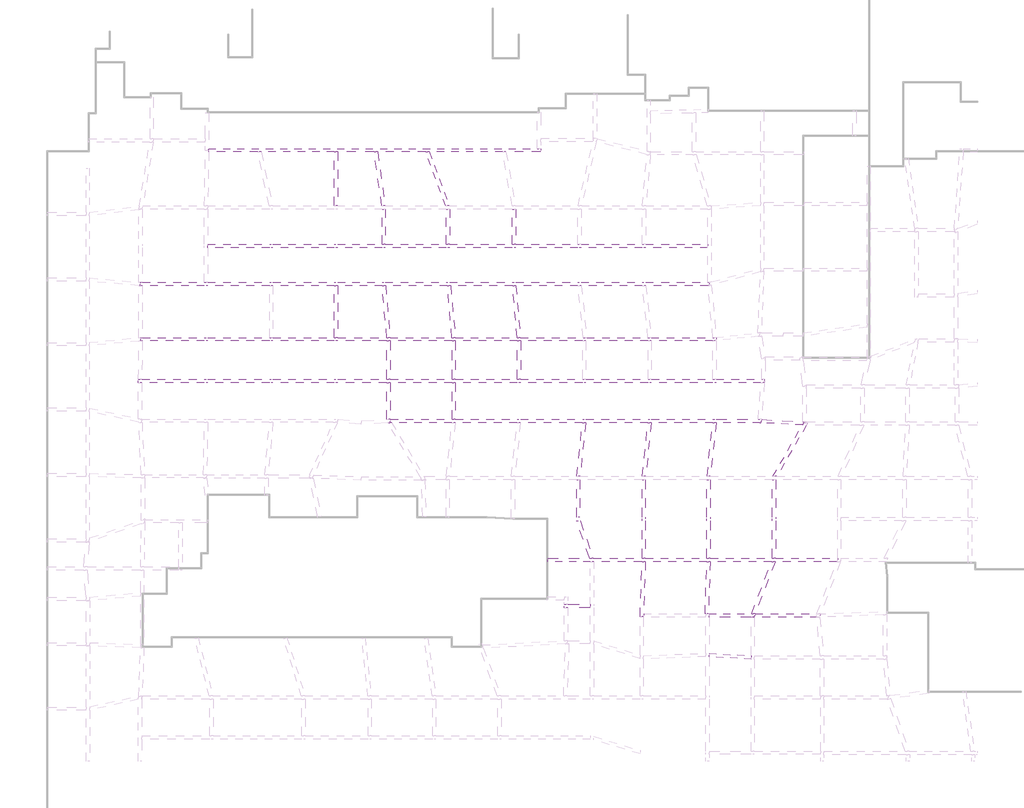
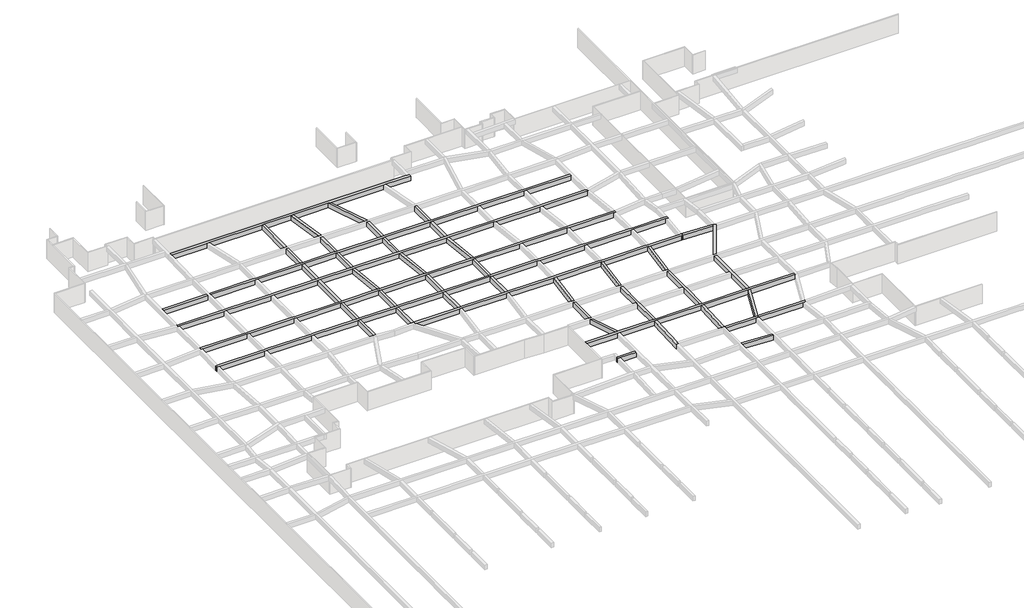
# One storey, part 36 of 45: 39 beams.
"""IFC4 building model written with IfcOpenShell, lengths in millimetres."""

from ifc_helpers import new_model, si_unit, frame, origin, place, context, project, spatial, polyline, outline, extrude, faceted_brep, element, save

model = new_model("IFC4")

# Units and contexts
model_context = context("Model", 3, world=origin())
ifc_project = project(units=[si_unit("LENGTHUNIT", "METRE", prefix="MILLI")], contexts=[model_context])

# Site, building, storey
site = spatial("IfcSite", under=ifc_project)
building = spatial("IfcBuilding", under=site)
storey = spatial("IfcBuildingStorey", under=building, Name="户型图", Elevation=0.0)

# Beams
placement = place(None, origin())
element("IfcBeam", 1, ObjectType="混凝土 - 矩形梁 : KL_beam", at=placement, inside=storey, context=model_context, shape_type="SweptSolid", body=[
    extrude(outline(polyline([(-120360.6744654, 184740.2921988), (-120760.6744654, 184740.2921988), (-120760.6744654, 191179.2504337), (-120360.6744654, 191179.2504337), (-120360.6744654, 184740.2921988)])), frame((0.0, 0.0, 2500.0), z_axis=(0.0, 0.0, 1.0), x_axis=(1.0, 0.0, 0.0)), (0.0, 0.0, 1.0), 800.0),
])
element("IfcBeam", 2, ObjectType="混凝土 - 矩形梁 : KL_beam", at=placement, inside=storey, context=model_context, shape_type="SweptSolid", body=[
    extrude(outline(polyline([(-114686.8171178, 184740.2921988), (-115090.7481468, 184740.2921988), (-115995.6847118, 191179.2504337), (-115591.7536828, 191179.2504337), (-114686.8171178, 184740.2921988)])), frame((0.0, 0.0, 2500.0), z_axis=(0.0, 0.0, 1.0), x_axis=(1.0, 0.0, 0.0)), (0.0, 0.0, 1.0), 800.0),
])
element("IfcBeam", 3, ObjectType="混凝土 - 矩形梁 : KL_beam", at=placement, inside=storey, context=model_context, shape_type="SweptSolid", body=[
    extrude(outline(polyline([(-107060.4801488, 184740.2921988), (-107486.1512578, 184740.2921988), (-109829.740395, 191179.2504337), (-109404.069286, 191179.2504337), (-107060.4801488, 184740.2921988)])), frame((0.0, 0.0, 2500.0), z_axis=(0.0, 0.0, 1.0), x_axis=(1.0, 0.0, 0.0)), (0.0, 0.0, 1.0), 800.0),
])
element("IfcBeam", 4, ObjectType="混凝土 - 矩形梁 : KL_beam", at=placement, inside=storey, context=model_context, shape_type="Brep", body=[
    faceted_brep([(-76031.325523, 175615.3210168, 3300.0), (-76160.6744654, 175615.3210168, 3300.0), (-83597.2475165, 175615.3210168, 3300.0), (-83997.2475165, 175615.3210168, 3300.0), (-91300.5216564, 175615.3210168, 3300.0), (-91700.5216564, 175615.3210168, 3300.0), (-99100.5216564, 175615.3210168, 3300.0), (-99500.5216564, 175615.3210168, 3300.0), (-107000.5216564, 175615.3210168, 3300.0), (-107400.5216564, 175615.3210168, 3300.0), (-114660.6744654, 175615.3210168, 3300.0), (-115060.6744654, 175615.3210168, 3300.0), (-120360.6744654, 175615.3210168, 3300.0), (-120760.6744654, 175615.3210168, 3300.0), (-128080.5216564, 175615.3210168, 3300.0), (-128480.5216564, 175615.3210168, 3300.0), (-135860.6744654, 175615.3210168, 3300.0), (-136260.6744654, 175615.3210168, 3300.0), (-143669.0135418, 175615.3210168, 3300.0), (-143895.9184786, 175615.3210168, 3300.0), (-143913.3828558, 175215.3210168, 3300.0), (-143669.0135418, 175215.3210168, 3300.0), (-136260.6744654, 175215.3210168, 3300.0), (-135860.6744654, 175215.3210168, 3300.0), (-128480.5216564, 175215.3210168, 3300.0), (-128080.5216564, 175215.3210168, 3300.0), (-120760.6744654, 175215.3210168, 3300.0), (-120360.6744654, 175215.3210168, 3300.0), (-115043.6071944, 175215.3210168, 3300.0), (-114642.0148509, 175215.3210168, 3300.0), (-107271.1801788, 175215.3210168, 3300.0), (-106869.5878353, 175215.3210168, 3300.0), (-99483.7878912, 175215.3210168, 3300.0), (-99082.2599562, 175215.3210168, 3300.0), (-91680.6024653, 175215.3210168, 3300.0), (-91278.3991535, 175215.3210168, 3300.0), (-83977.3283253, 175215.3210168, 3300.0), (-83575.1250135, 175215.3210168, 3300.0), (-76142.4560482, 175215.3210168, 3300.0), (-75977.9758113, 175215.3210168, 3300.0), (-143913.3828558, 175215.3210168, 2500.0), (-143669.0135418, 175215.3210168, 2500.0), (-136260.6744654, 175215.3210168, 2500.0), (-135860.6744654, 175215.3210168, 2500.0), (-128480.5216564, 175215.3210168, 2500.0), (-128080.5216564, 175215.3210168, 2500.0), (-120760.6744654, 175215.3210168, 2500.0), (-120360.6744654, 175215.3210168, 2500.0), (-115043.6071944, 175215.3210168, 2500.0), (-114642.0148509, 175215.3210168, 2500.0), (-107271.1801788, 175215.3210168, 2500.0), (-106869.5878353, 175215.3210168, 2500.0), (-99483.7878912, 175215.3210168, 2500.0), (-99082.2599562, 175215.3210168, 2500.0), (-91680.6024653, 175215.3210168, 2500.0), (-91278.3991535, 175215.3210168, 2500.0), (-83977.3283253, 175215.3210168, 2500.0), (-83575.1250135, 175215.3210168, 2500.0), (-76142.4560482, 175215.3210168, 2500.0), (-75977.9758113, 175215.3210168, 2500.0), (-143895.9184786, 175615.3210168, 2500.0), (-143669.0135418, 175615.3210168, 2500.0), (-136260.6744654, 175615.3210168, 2500.0), (-135860.6744654, 175615.3210168, 2500.0), (-128480.5216564, 175615.3210168, 2500.0), (-128080.5216564, 175615.3210168, 2500.0), (-120760.6744654, 175615.3210168, 2500.0), (-120360.6744654, 175615.3210168, 2500.0), (-115060.6744654, 175615.3210168, 2500.0), (-114660.6744654, 175615.3210168, 2500.0), (-107400.5216564, 175615.3210168, 2500.0), (-107000.5216564, 175615.3210168, 2500.0), (-99500.5216564, 175615.3210168, 2500.0), (-99100.5216564, 175615.3210168, 2500.0), (-91700.5216564, 175615.3210168, 2500.0), (-91300.5216564, 175615.3210168, 2500.0), (-83997.2475165, 175615.3210168, 2500.0), (-83597.2475165, 175615.3210168, 2500.0), (-76160.6744654, 175615.3210168, 2500.0), (-76031.325523, 175615.3210168, 2500.0)], [[[0, 1, 2, 3, 4, 5, 6, 7, 8, 9, 10, 11, 12, 13, 14, 15, 16, 17, 18, 19, 20, 21, 22, 23, 24, 25, 26, 27, 28, 29, 30, 31, 32, 33, 34, 35, 36, 37, 38, 39]], [[39, 38, 37, 36, 35, 34, 33, 32, 31, 30, 29, 28, 27, 26, 25, 24, 23, 22, 21, 20, 40, 41, 42, 43, 44, 45, 46, 47, 48, 49, 50, 51, 52, 53, 54, 55, 56, 57, 58, 59]], [[59, 58, 57, 56, 55, 54, 53, 52, 51, 50, 49, 48, 47, 46, 45, 44, 43, 42, 41, 40, 60, 61, 62, 63, 64, 65, 66, 67, 68, 69, 70, 71, 72, 73, 74, 75, 76, 77, 78, 79]], [[19, 18, 17, 16, 15, 14, 13, 12, 11, 10, 9, 8, 7, 6, 5, 4, 3, 2, 1, 0, 79, 78, 77, 76, 75, 74, 73, 72, 71, 70, 69, 68, 67, 66, 65, 64, 63, 62, 61, 60]], [[19, 60, 40, 20]], [[0, 39, 59, 79]]]),
])
element("IfcBeam", 5, ObjectType="混凝土 - 矩形梁 : KL_beam", at=placement, inside=storey, context=model_context, shape_type="Brep", body=[
    faceted_brep([(-75186.161196, 169035.1135794, 3300.0), (-75587.7690547, 169035.1135794, 3300.0), (-82925.559037, 169035.1135794, 3300.0), (-83327.7623488, 169035.1135794, 3300.0), (-90628.833177, 169035.1135794, 3300.0), (-91031.0364888, 169035.1135794, 3300.0), (-98541.5618672, 169035.1135794, 3300.0), (-98943.0898022, 169035.1135794, 3300.0), (-106317.5889274, 169035.1135794, 3300.0), (-106719.1812709, 169035.1135794, 3300.0), (-114090.0159431, 169035.1135794, 3300.0), (-114491.6082865, 169035.1135794, 3300.0), (-120360.6744654, 169035.1135794, 3300.0), (-120760.6744654, 169035.1135794, 3300.0), (-128080.5216564, 169035.1135794, 3300.0), (-128480.5216564, 169035.1135794, 3300.0), (-135860.6744654, 169035.1135794, 3300.0), (-136260.6744654, 169035.1135794, 3300.0), (-143669.0135418, 169035.1135794, 3300.0), (-143878.581976, 169035.1135794, 3300.0), (-143859.4474089, 168635.1135794, 3300.0), (-143671.4793509, 168635.1135794, 3300.0), (-136260.6744654, 168635.1135794, 3300.0), (-135860.6744654, 168635.1135794, 3300.0), (-128480.5216564, 168635.1135794, 3300.0), (-128080.5216564, 168635.1135794, 3300.0), (-120760.6744654, 168635.1135794, 3300.0), (-120360.6744654, 168635.1135794, 3300.0), (-114472.9294157, 168635.1135794, 3300.0), (-114072.9294157, 168635.1135794, 3300.0), (-106700.5216564, 168635.1135794, 3300.0), (-106300.5216564, 168635.1135794, 3300.0), (-98924.7994609, 168635.1135794, 3300.0), (-98524.7994609, 168635.1135794, 3300.0), (-91124.7994609, 168635.1135794, 3300.0), (-90724.7994609, 168635.1135794, 3300.0), (-83305.6398459, 168635.1135794, 3300.0), (-82905.6398459, 168635.1135794, 3300.0), (-75569.0146925, 168635.1135794, 3300.0), (-75358.5331366, 168635.1135794, 3300.0), (-75186.161196, 168635.1135794, 3300.0), (-75186.161196, 168653.2306004, 3300.0), (-143859.4474089, 168635.1135794, 2500.0), (-143671.4793509, 168635.1135794, 2500.0), (-136260.6744654, 168635.1135794, 2500.0), (-135860.6744654, 168635.1135794, 2500.0), (-128480.5216564, 168635.1135794, 2500.0), (-128080.5216564, 168635.1135794, 2500.0), (-120760.6744654, 168635.1135794, 2500.0), (-120360.6744654, 168635.1135794, 2500.0), (-114472.9294157, 168635.1135794, 2500.0), (-114072.9294157, 168635.1135794, 2500.0), (-106700.5216564, 168635.1135794, 2500.0), (-106300.5216564, 168635.1135794, 2500.0), (-98924.7994609, 168635.1135794, 2500.0), (-98524.7994609, 168635.1135794, 2500.0), (-91124.7994609, 168635.1135794, 2500.0), (-90724.7994609, 168635.1135794, 2500.0), (-83305.6398459, 168635.1135794, 2500.0), (-82905.6398459, 168635.1135794, 2500.0), (-75569.0146925, 168635.1135794, 2500.0), (-75358.5331366, 168635.1135794, 2500.0), (-75186.161196, 168635.1135794, 2500.0), (-143878.581976, 169035.1135794, 2500.0), (-143669.0135418, 169035.1135794, 2500.0), (-136260.6744654, 169035.1135794, 2500.0), (-135860.6744654, 169035.1135794, 2500.0), (-128480.5216564, 169035.1135794, 2500.0), (-128080.5216564, 169035.1135794, 2500.0), (-120760.6744654, 169035.1135794, 2500.0), (-120360.6744654, 169035.1135794, 2500.0), (-114491.6082865, 169035.1135794, 2500.0), (-114090.0159431, 169035.1135794, 2500.0), (-106719.1812709, 169035.1135794, 2500.0), (-106317.5889274, 169035.1135794, 2500.0), (-98943.0898022, 169035.1135794, 2500.0), (-98541.5618672, 169035.1135794, 2500.0), (-91031.0364888, 169035.1135794, 2500.0), (-90628.833177, 169035.1135794, 2500.0), (-83327.7623488, 169035.1135794, 2500.0), (-82925.559037, 169035.1135794, 2500.0), (-75587.7690547, 169035.1135794, 2500.0), (-75186.161196, 169035.1135794, 2500.0), (-75186.161196, 168653.2306004, 2500.0)], [[[0, 1, 2, 3, 4, 5, 6, 7, 8, 9, 10, 11, 12, 13, 14, 15, 16, 17, 18, 19, 20, 21, 22, 23, 24, 25, 26, 27, 28, 29, 30, 31, 32, 33, 34, 35, 36, 37, 38, 39, 40, 41]], [[40, 39, 38, 37, 36, 35, 34, 33, 32, 31, 30, 29, 28, 27, 26, 25, 24, 23, 22, 21, 20, 42, 43, 44, 45, 46, 47, 48, 49, 50, 51, 52, 53, 54, 55, 56, 57, 58, 59, 60, 61, 62]], [[62, 61, 60, 59, 58, 57, 56, 55, 54, 53, 52, 51, 50, 49, 48, 47, 46, 45, 44, 43, 42, 63, 64, 65, 66, 67, 68, 69, 70, 71, 72, 73, 74, 75, 76, 77, 78, 79, 80, 81, 82, 83]], [[19, 18, 17, 16, 15, 14, 13, 12, 11, 10, 9, 8, 7, 6, 5, 4, 3, 2, 1, 0, 82, 81, 80, 79, 78, 77, 76, 75, 74, 73, 72, 71, 70, 69, 68, 67, 66, 65, 64, 63]], [[19, 63, 42, 20]], [[0, 41, 40, 62, 83, 82]]]),
])
element("IfcBeam", 6, ObjectType="混凝土 - 矩形梁 : KL_beam", at=placement, inside=storey, context=model_context, shape_type="Brep", body=[
    faceted_brep([(-69444.6043733, 163650.6823883, 3300.0), (-69444.6043733, 163735.2368527, 3300.0), (-69444.6043733, 164050.6823883, 3300.0), (-69744.9443936, 164050.6823883, 3300.0), (-75169.0146925, 164050.6823883, 3300.0), (-75569.0146925, 164050.6823883, 3300.0), (-82905.6398459, 164050.6823883, 3300.0), (-83305.6398459, 164050.6823883, 3300.0), (-90724.7994609, 164050.6823883, 3300.0), (-91124.7994609, 164050.6823883, 3300.0), (-98524.7994609, 164050.6823883, 3300.0), (-98924.7994609, 164050.6823883, 3300.0), (-106300.5216564, 164050.6823883, 3300.0), (-106700.5216564, 164050.6823883, 3300.0), (-114072.9294157, 164050.6823883, 3300.0), (-114472.9294157, 164050.6823883, 3300.0), (-120360.6744654, 164050.6823883, 3300.0), (-120760.6744654, 164050.6823883, 3300.0), (-128080.5216564, 164050.6823883, 3300.0), (-128480.5216564, 164050.6823883, 3300.0), (-135860.6744654, 164050.6823883, 3300.0), (-136260.6744654, 164050.6823883, 3300.0), (-143728.3270835, 164050.6823883, 3300.0), (-144128.3578352, 164050.6823883, 3300.0), (-144130.8224936, 164050.6823883, 3300.0), (-144130.8224936, 163650.6823883, 3300.0), (-143730.8224936, 163650.6823883, 3300.0), (-136260.6744654, 163650.6823883, 3300.0), (-135860.6744654, 163650.6823883, 3300.0), (-128480.5216564, 163650.6823883, 3300.0), (-128080.5216564, 163650.6823883, 3300.0), (-120760.6744654, 163650.6823883, 3300.0), (-120360.6744654, 163650.6823883, 3300.0), (-114472.9294157, 163650.6823883, 3300.0), (-114072.9294157, 163650.6823883, 3300.0), (-106700.5216564, 163650.6823883, 3300.0), (-106300.5216564, 163650.6823883, 3300.0), (-98924.7994609, 163650.6823883, 3300.0), (-98524.7994609, 163650.6823883, 3300.0), (-91124.7994609, 163650.6823883, 3300.0), (-90724.7994609, 163650.6823883, 3300.0), (-83305.6398459, 163650.6823883, 3300.0), (-82905.6398459, 163650.6823883, 3300.0), (-75569.0146925, 163650.6823883, 3300.0), (-75169.0146925, 163650.6823883, 3300.0), (-69845.6243611, 163650.6823883, 3300.0), (-69444.6043733, 163650.6823883, 2500.0), (-144130.8224936, 163650.6823883, 2500.0), (-143730.8224936, 163650.6823883, 2500.0), (-136260.6744654, 163650.6823883, 2500.0), (-135860.6744654, 163650.6823883, 2500.0), (-128480.5216564, 163650.6823883, 2500.0), (-128080.5216564, 163650.6823883, 2500.0), (-120760.6744654, 163650.6823883, 2500.0), (-120360.6744654, 163650.6823883, 2500.0), (-114472.9294157, 163650.6823883, 2500.0), (-114072.9294157, 163650.6823883, 2500.0), (-106700.5216564, 163650.6823883, 2500.0), (-106300.5216564, 163650.6823883, 2500.0), (-98924.7994609, 163650.6823883, 2500.0), (-98524.7994609, 163650.6823883, 2500.0), (-91124.7994609, 163650.6823883, 2500.0), (-90724.7994609, 163650.6823883, 2500.0), (-83305.6398459, 163650.6823883, 2500.0), (-82905.6398459, 163650.6823883, 2500.0), (-75569.0146925, 163650.6823883, 2500.0), (-75169.0146925, 163650.6823883, 2500.0), (-69845.6243611, 163650.6823883, 2500.0), (-69444.6043733, 164050.6823883, 2500.0), (-69444.6043733, 163735.2368527, 2500.0), (-144130.8224936, 164050.6823883, 2500.0), (-144128.3578352, 164050.6823883, 2500.0), (-143728.3270835, 164050.6823883, 2500.0), (-136260.6744654, 164050.6823883, 2500.0), (-135860.6744654, 164050.6823883, 2500.0), (-128480.5216564, 164050.6823883, 2500.0), (-128080.5216564, 164050.6823883, 2500.0), (-120760.6744654, 164050.6823883, 2500.0), (-120360.6744654, 164050.6823883, 2500.0), (-114472.9294157, 164050.6823883, 2500.0), (-114072.9294157, 164050.6823883, 2500.0), (-106700.5216564, 164050.6823883, 2500.0), (-106300.5216564, 164050.6823883, 2500.0), (-98924.7994609, 164050.6823883, 2500.0), (-98524.7994609, 164050.6823883, 2500.0), (-91124.7994609, 164050.6823883, 2500.0), (-90724.7994609, 164050.6823883, 2500.0), (-83305.6398459, 164050.6823883, 2500.0), (-82905.6398459, 164050.6823883, 2500.0), (-75569.0146925, 164050.6823883, 2500.0), (-75169.0146925, 164050.6823883, 2500.0), (-69744.9443936, 164050.6823883, 2500.0)], [[[0, 1, 2, 3, 4, 5, 6, 7, 8, 9, 10, 11, 12, 13, 14, 15, 16, 17, 18, 19, 20, 21, 22, 23, 24, 25, 26, 27, 28, 29, 30, 31, 32, 33, 34, 35, 36, 37, 38, 39, 40, 41, 42, 43, 44, 45]], [[46, 0, 45, 44, 43, 42, 41, 40, 39, 38, 37, 36, 35, 34, 33, 32, 31, 30, 29, 28, 27, 26, 25, 47, 48, 49, 50, 51, 52, 53, 54, 55, 56, 57, 58, 59, 60, 61, 62, 63, 64, 65, 66, 67]], [[68, 69, 46, 67, 66, 65, 64, 63, 62, 61, 60, 59, 58, 57, 56, 55, 54, 53, 52, 51, 50, 49, 48, 47, 70, 71, 72, 73, 74, 75, 76, 77, 78, 79, 80, 81, 82, 83, 84, 85, 86, 87, 88, 89, 90, 91]], [[2, 68, 91, 90, 89, 88, 87, 86, 85, 84, 83, 82, 81, 80, 79, 78, 77, 76, 75, 74, 73, 72, 71, 70, 24, 23, 22, 21, 20, 19, 18, 17, 16, 15, 14, 13, 12, 11, 10, 9, 8, 7, 6, 5, 4, 3]], [[25, 24, 70, 47]], [[2, 1, 0, 46, 69, 68]]]),
])
element("IfcBeam", 7, ObjectType="混凝土 - 矩形梁 : KL_beam", at=placement, inside=storey, context=model_context, shape_type="Brep", body=[
    faceted_brep([(-143669.0135418, 180177.2946529, 3300.0), (-143669.0135418, 179777.2946529, 3300.0), (-136260.6744654, 179777.2946529, 3300.0), (-136260.6744654, 180177.2946529, 3300.0), (-143669.0135418, 179777.2946529, 2500.0), (-136260.6744654, 179777.2946529, 2500.0), (-143669.0135418, 180177.2946529, 2500.0), (-136260.6744654, 180177.2946529, 2500.0)], [[[0, 1, 2, 3]], [[1, 4, 5, 2]], [[4, 6, 7, 5]], [[6, 0, 3, 7]], [[1, 0, 6, 4]], [[3, 2, 5, 7]]]),
    faceted_brep([(-135860.6744654, 179777.2946529, 3300.0), (-135860.6744654, 180177.2946529, 3300.0), (-135860.6744654, 180177.2946529, 2500.0), (-135860.6744654, 179777.2946529, 2500.0), (-128480.5216564, 179777.2946529, 3300.0), (-128080.5216564, 179777.2946529, 3300.0), (-120760.6744654, 179777.2946529, 3300.0), (-120360.6744654, 179777.2946529, 3300.0), (-115060.6744654, 179777.2946529, 3300.0), (-114660.6744654, 179777.2946529, 3300.0), (-107400.5216564, 179777.2946529, 3300.0), (-107000.5216564, 179777.2946529, 3300.0), (-99500.5216564, 179777.2946529, 3300.0), (-99100.5216564, 179777.2946529, 3300.0), (-91700.5216564, 179777.2946529, 3300.0), (-91300.5216564, 179777.2946529, 3300.0), (-83997.2475165, 179777.2946529, 3300.0), (-83597.2475165, 179777.2946529, 3300.0), (-76160.6744654, 179777.2946529, 3300.0), (-76160.6744654, 180177.2946529, 3300.0), (-83597.2475165, 180177.2946529, 3300.0), (-83997.2475165, 180177.2946529, 3300.0), (-91300.5216564, 180177.2946529, 3300.0), (-91700.5216564, 180177.2946529, 3300.0), (-99100.5216564, 180177.2946529, 3300.0), (-99500.5216564, 180177.2946529, 3300.0), (-107000.5216564, 180177.2946529, 3300.0), (-107400.5216564, 180177.2946529, 3300.0), (-114660.6744654, 180177.2946529, 3300.0), (-115060.6744654, 180177.2946529, 3300.0), (-120360.6744654, 180177.2946529, 3300.0), (-120760.6744654, 180177.2946529, 3300.0), (-128080.5216564, 180177.2946529, 3300.0), (-128480.5216564, 180177.2946529, 3300.0), (-128480.5216564, 179777.2946529, 2500.0), (-128080.5216564, 179777.2946529, 2500.0), (-120760.6744654, 179777.2946529, 2500.0), (-120360.6744654, 179777.2946529, 2500.0), (-115060.6744654, 179777.2946529, 2500.0), (-114660.6744654, 179777.2946529, 2500.0), (-107400.5216564, 179777.2946529, 2500.0), (-107000.5216564, 179777.2946529, 2500.0), (-99500.5216564, 179777.2946529, 2500.0), (-99100.5216564, 179777.2946529, 2500.0), (-91700.5216564, 179777.2946529, 2500.0), (-91300.5216564, 179777.2946529, 2500.0), (-83997.2475165, 179777.2946529, 2500.0), (-83597.2475165, 179777.2946529, 2500.0), (-76160.6744654, 179777.2946529, 2500.0), (-128480.5216564, 180177.2946529, 2500.0), (-128080.5216564, 180177.2946529, 2500.0), (-120760.6744654, 180177.2946529, 2500.0), (-120360.6744654, 180177.2946529, 2500.0), (-115060.6744654, 180177.2946529, 2500.0), (-114660.6744654, 180177.2946529, 2500.0), (-107400.5216564, 180177.2946529, 2500.0), (-107000.5216564, 180177.2946529, 2500.0), (-99500.5216564, 180177.2946529, 2500.0), (-99100.5216564, 180177.2946529, 2500.0), (-91700.5216564, 180177.2946529, 2500.0), (-91300.5216564, 180177.2946529, 2500.0), (-83997.2475165, 180177.2946529, 2500.0), (-83597.2475165, 180177.2946529, 2500.0), (-76160.6744654, 180177.2946529, 2500.0)], [[[0, 1, 2, 3]], [[1, 0, 4, 5, 6, 7, 8, 9, 10, 11, 12, 13, 14, 15, 16, 17, 18, 19, 20, 21, 22, 23, 24, 25, 26, 27, 28, 29, 30, 31, 32, 33]], [[0, 3, 34, 35, 36, 37, 38, 39, 40, 41, 42, 43, 44, 45, 46, 47, 48, 18, 17, 16, 15, 14, 13, 12, 11, 10, 9, 8, 7, 6, 5, 4]], [[3, 2, 49, 50, 51, 52, 53, 54, 55, 56, 57, 58, 59, 60, 61, 62, 63, 48, 47, 46, 45, 44, 43, 42, 41, 40, 39, 38, 37, 36, 35, 34]], [[2, 1, 33, 32, 31, 30, 29, 28, 27, 26, 25, 24, 23, 22, 21, 20, 19, 63, 62, 61, 60, 59, 58, 57, 56, 55, 54, 53, 52, 51, 50, 49]], [[19, 18, 48, 63]]]),
])
element("IfcBeam", 8, ObjectType="混凝土 - 矩形梁 : KL_beam", at=placement, inside=storey, context=model_context, shape_type="SweptSolid", body=[
    extrude(outline(polyline([(-120760.6744654, 184340.2921988), (-120360.6744654, 184340.2921988), (-120360.6744654, 180177.2946529), (-120760.6744654, 180177.2946529), (-120760.6744654, 184340.2921988)])), frame((0.0, 0.0, 2500.0), z_axis=(0.0, 0.0, 1.0), x_axis=(1.0, 0.0, 0.0)), (0.0, 0.0, 1.0), 800.0),
    extrude(outline(polyline([(-120360.6744654, 159299.3775215), (-120760.6744654, 159299.3775215), (-120760.6744654, 163650.6823883), (-120360.6744654, 163650.6823883), (-120360.6744654, 159299.3775215)])), frame((0.0, 0.0, 2500.0), z_axis=(0.0, 0.0, 1.0), x_axis=(1.0, 0.0, 0.0)), (0.0, 0.0, 1.0), 800.0),
    extrude(outline(polyline([(-120760.6744654, 175215.3210168), (-120360.6744654, 175215.3210168), (-120360.6744654, 169035.1135794), (-120760.6744654, 169035.1135794), (-120760.6744654, 175215.3210168)])), frame((0.0, 0.0, 2500.0), z_axis=(0.0, 0.0, 1.0), x_axis=(1.0, 0.0, 0.0)), (0.0, 0.0, 1.0), 800.0),
    extrude(outline(polyline([(-120360.6744654, 175615.3210168), (-120760.6744654, 175615.3210168), (-120760.6744654, 179777.2946529), (-120360.6744654, 179777.2946529), (-120360.6744654, 175615.3210168)])), frame((0.0, 0.0, 2500.0), z_axis=(0.0, 0.0, 1.0), x_axis=(1.0, 0.0, 0.0)), (0.0, 0.0, 1.0), 800.0),
    extrude(outline(polyline([(-120760.6744654, 168635.1135794), (-120360.6744654, 168635.1135794), (-120360.6744654, 164050.6823883), (-120760.6744654, 164050.6823883), (-120760.6744654, 168635.1135794)])), frame((0.0, 0.0, 2500.0), z_axis=(0.0, 0.0, 1.0), x_axis=(1.0, 0.0, 0.0)), (0.0, 0.0, 1.0), 800.0),
])
element("IfcBeam", 9, ObjectType="混凝土 - 矩形梁 : KL_beam", at=placement, inside=storey, context=model_context, shape_type="SweptSolid", body=[
    extrude(outline(polyline([(-114072.9294157, 159273.5727809), (-114472.9294157, 159252.6096692), (-114472.9294157, 163650.6823883), (-114072.9294157, 163650.6823883), (-114072.9294157, 159273.5727809)])), frame((0.0, 0.0, 2500.0), z_axis=(0.0, 0.0, 1.0), x_axis=(1.0, 0.0, 0.0)), (0.0, 0.0, 1.0), 800.0),
])
element("IfcBeam", 10, ObjectType="混凝土 - 矩形梁 : KL_beam", at=placement, inside=storey, context=model_context, shape_type="SweptSolid", body=[
    extrude(outline(polyline([(-114472.9294157, 168635.1135794), (-114072.9294157, 168635.1135794), (-114072.9294157, 164050.6823883), (-114472.9294157, 164050.6823883), (-114472.9294157, 168635.1135794)])), frame((0.0, 0.0, 2500.0), z_axis=(0.0, 0.0, 1.0), x_axis=(1.0, 0.0, 0.0)), (0.0, 0.0, 1.0), 800.0),
])
element("IfcBeam", 11, ObjectType="混凝土 - 矩形梁 : KL_beam", at=placement, inside=storey, context=model_context, shape_type="SweptSolid", body=[
    extrude(outline(polyline([(-115060.6744654, 184340.2921988), (-114660.6744654, 184340.2921988), (-114660.6744654, 180177.2946529), (-115060.6744654, 180177.2946529), (-115060.6744654, 184340.2921988)])), frame((0.0, 0.0, 2500.0), z_axis=(0.0, 0.0, 1.0), x_axis=(1.0, 0.0, 0.0)), (0.0, 0.0, 1.0), 800.0),
    extrude(outline(polyline([(-114660.6744654, 175615.3210168), (-115060.6744654, 175615.3210168), (-115060.6744654, 179777.2946529), (-114660.6744654, 179777.2946529), (-114660.6744654, 175615.3210168)])), frame((0.0, 0.0, 2500.0), z_axis=(0.0, 0.0, 1.0), x_axis=(1.0, 0.0, 0.0)), (0.0, 0.0, 1.0), 800.0),
])
element("IfcBeam", 12, ObjectType="混凝土 - 矩形梁 : KL_beam", at=placement, inside=storey, context=model_context, shape_type="SweptSolid", body=[
    extrude(outline(polyline([(-115043.6071944, 175215.3210168), (-114642.0148509, 175215.3210168), (-114090.0159431, 169035.1135794), (-114491.6082865, 169035.1135794), (-115043.6071944, 175215.3210168)])), frame((0.0, 0.0, 2500.0), z_axis=(0.0, 0.0, 1.0), x_axis=(1.0, 0.0, 0.0)), (0.0, 0.0, 1.0), 800.0),
])
element("IfcBeam", 13, ObjectType="混凝土 - 矩形梁 : KL_beam", at=placement, inside=storey, context=model_context, shape_type="SweptSolid", body=[
    extrude(outline(polyline([(-107400.5216564, 184340.2921988), (-107000.5216564, 184340.2921988), (-107000.5216564, 180177.2946529), (-107400.5216564, 180177.2946529), (-107400.5216564, 184340.2921988)])), frame((0.0, 0.0, 2500.0), z_axis=(0.0, 0.0, 1.0), x_axis=(1.0, 0.0, 0.0)), (0.0, 0.0, 1.0), 800.0),
    extrude(outline(polyline([(-107000.5216564, 175615.3210168), (-107400.5216564, 175615.3210168), (-107400.5216564, 179777.2946529), (-107000.5216564, 179777.2946529), (-107000.5216564, 175615.3210168)])), frame((0.0, 0.0, 2500.0), z_axis=(0.0, 0.0, 1.0), x_axis=(1.0, 0.0, 0.0)), (0.0, 0.0, 1.0), 800.0),
])
element("IfcBeam", 14, ObjectType="混凝土 - 矩形梁 : KL_beam", at=placement, inside=storey, context=model_context, shape_type="SweptSolid", body=[
    extrude(outline(polyline([(-107271.1801788, 175215.3210168), (-106869.5878353, 175215.3210168), (-106317.5889274, 169035.1135794), (-106719.1812709, 169035.1135794), (-107271.1801788, 175215.3210168)])), frame((0.0, 0.0, 2500.0), z_axis=(0.0, 0.0, 1.0), x_axis=(1.0, 0.0, 0.0)), (0.0, 0.0, 1.0), 800.0),
])
element("IfcBeam", 15, ObjectType="混凝土 - 矩形梁 : KL_beam", at=placement, inside=storey, context=model_context, shape_type="SweptSolid", body=[
    extrude(outline(polyline([(-106700.5216564, 168635.1135794), (-106300.5216564, 168635.1135794), (-106300.5216564, 164050.6823883), (-106700.5216564, 164050.6823883), (-106700.5216564, 168635.1135794)])), frame((0.0, 0.0, 2500.0), z_axis=(0.0, 0.0, 1.0), x_axis=(1.0, 0.0, 0.0)), (0.0, 0.0, 1.0), 800.0),
])
element("IfcBeam", 16, ObjectType="混凝土 - 矩形梁 : KL_beam", at=placement, inside=storey, context=model_context, shape_type="SweptSolid", body=[
    extrude(outline(polyline([(-106700.5216564, 163650.6823883), (-106300.5216564, 163650.6823883), (-106300.5216564, 159263.2495721), (-106700.5216564, 159263.2495721), (-106700.5216564, 163650.6823883)])), frame((0.0, 0.0, 2500.0), z_axis=(0.0, 0.0, 1.0), x_axis=(1.0, 0.0, 0.0)), (0.0, 0.0, 1.0), 800.0),
])
element("IfcBeam", 17, ObjectType="混凝土 - 矩形梁 : KL_beam", at=placement, inside=storey, context=model_context, shape_type="Brep", body=[
    faceted_brep([(-114072.9294157, 159263.2495721, 3300.0), (-114072.9294157, 158873.0238425, 3300.0), (-114259.4336062, 158863.2495721, 3300.0), (-113919.6906746, 158863.2495721, 3300.0), (-106722.8306205, 158863.2495721, 3300.0), (-106320.5918899, 158863.2495721, 3300.0), (-98947.1541949, 158863.2495721, 3300.0), (-98544.9154643, 158863.2495721, 3300.0), (-91147.1541949, 158863.2495721, 3300.0), (-90744.9154643, 158863.2495721, 3300.0), (-83327.9488099, 158863.2495721, 3300.0), (-82925.7100793, 158863.2495721, 3300.0), (-75591.3694264, 158863.2495721, 3300.0), (-75189.1306958, 158863.2495721, 3300.0), (-69978.1666, 158863.2495721, 3300.0), (-69786.7112953, 158863.2495721, 3300.0), (-69758.9094454, 159252.3077299, 3300.0), (-69758.1275482, 159263.2495721, 3300.0), (-70159.147536, 159263.2495721, 3300.0), (-75169.0146925, 159263.2495721, 3300.0), (-75569.0146925, 159263.2495721, 3300.0), (-82905.6398459, 159263.2495721, 3300.0), (-83305.6398459, 159263.2495721, 3300.0), (-90724.7994609, 159263.2495721, 3300.0), (-91124.7994609, 159263.2495721, 3300.0), (-98524.7994609, 159263.2495721, 3300.0), (-98924.7994609, 159263.2495721, 3300.0), (-106300.5216564, 159263.2495721, 3300.0), (-106700.5216564, 159263.2495721, 3300.0), (-114259.4336062, 158863.2495721, 2500.0), (-113919.6906746, 158863.2495721, 2500.0), (-106722.8306205, 158863.2495721, 2500.0), (-106320.5918899, 158863.2495721, 2500.0), (-98947.1541949, 158863.2495721, 2500.0), (-98544.9154643, 158863.2495721, 2500.0), (-91147.1541949, 158863.2495721, 2500.0), (-90744.9154643, 158863.2495721, 2500.0), (-83327.9488099, 158863.2495721, 2500.0), (-82925.7100793, 158863.2495721, 2500.0), (-75591.3694264, 158863.2495721, 2500.0), (-75189.1306958, 158863.2495721, 2500.0), (-69978.1666, 158863.2495721, 2500.0), (-69786.7112953, 158863.2495721, 2500.0), (-114072.9294157, 158873.0238425, 2500.0), (-114072.9294157, 159263.2495721, 2500.0), (-106700.5216564, 159263.2495721, 2500.0), (-106300.5216564, 159263.2495721, 2500.0), (-98924.7994609, 159263.2495721, 2500.0), (-98524.7994609, 159263.2495721, 2500.0), (-91124.7994609, 159263.2495721, 2500.0), (-90724.7994609, 159263.2495721, 2500.0), (-83305.6398459, 159263.2495721, 2500.0), (-82905.6398459, 159263.2495721, 2500.0), (-75569.0146925, 159263.2495721, 2500.0), (-75169.0146925, 159263.2495721, 2500.0), (-70159.147536, 159263.2495721, 2500.0), (-69758.1275482, 159263.2495721, 2500.0), (-69758.9094454, 159252.3077299, 2500.0)], [[[0, 1, 2, 3, 4, 5, 6, 7, 8, 9, 10, 11, 12, 13, 14, 15, 16, 17, 18, 19, 20, 21, 22, 23, 24, 25, 26, 27, 28]], [[2, 29, 30, 31, 32, 33, 34, 35, 36, 37, 38, 39, 40, 41, 42, 15, 14, 13, 12, 11, 10, 9, 8, 7, 6, 5, 4, 3]], [[43, 44, 45, 46, 47, 48, 49, 50, 51, 52, 53, 54, 55, 56, 57, 42, 41, 40, 39, 38, 37, 36, 35, 34, 33, 32, 31, 30, 29]], [[44, 0, 28, 27, 26, 25, 24, 23, 22, 21, 20, 19, 18, 17, 56, 55, 54, 53, 52, 51, 50, 49, 48, 47, 46, 45]], [[43, 1, 0, 44]], [[1, 43, 29, 2]], [[17, 16, 15, 42, 57, 56]]]),
])
element("IfcBeam", 18, ObjectType="混凝土 - 矩形梁 : KL_beam", at=placement, inside=storey, context=model_context, shape_type="SweptSolid", body=[
    extrude(outline(polyline([(-99500.5216564, 184340.2921988), (-99100.5216564, 184340.2921988), (-99100.5216564, 180177.2946529), (-99500.5216564, 180177.2946529), (-99500.5216564, 184340.2921988)])), frame((0.0, 0.0, 2500.0), z_axis=(0.0, 0.0, 1.0), x_axis=(1.0, 0.0, 0.0)), (0.0, 0.0, 1.0), 800.0),
    extrude(outline(polyline([(-99100.5216564, 175615.3210168), (-99500.5216564, 175615.3210168), (-99500.5216564, 179777.2946529), (-99100.5216564, 179777.2946529), (-99100.5216564, 175615.3210168)])), frame((0.0, 0.0, 2500.0), z_axis=(0.0, 0.0, 1.0), x_axis=(1.0, 0.0, 0.0)), (0.0, 0.0, 1.0), 800.0),
])
element("IfcBeam", 19, ObjectType="混凝土 - 矩形梁 : KL_beam", at=placement, inside=storey, context=model_context, shape_type="SweptSolid", body=[
    extrude(outline(polyline([(-99483.7878912, 175215.3210168), (-99082.2599562, 175215.3210168), (-98541.5618672, 169035.1135794), (-98943.0898022, 169035.1135794), (-99483.7878912, 175215.3210168)])), frame((0.0, 0.0, 2500.0), z_axis=(0.0, 0.0, 1.0), x_axis=(1.0, 0.0, 0.0)), (0.0, 0.0, 1.0), 800.0),
])
element("IfcBeam", 20, ObjectType="混凝土 - 矩形梁 : KL_beam", at=placement, inside=storey, context=model_context, shape_type="SweptSolid", body=[
    extrude(outline(polyline([(-98924.7994609, 168635.1135794), (-98524.7994609, 168635.1135794), (-98524.7994609, 164050.6823883), (-98924.7994609, 164050.6823883), (-98924.7994609, 168635.1135794)])), frame((0.0, 0.0, 2500.0), z_axis=(0.0, 0.0, 1.0), x_axis=(1.0, 0.0, 0.0)), (0.0, 0.0, 1.0), 800.0),
    extrude(outline(polyline([(-98524.7994609, 159263.2495721), (-98924.7994609, 159263.2495721), (-98924.7994609, 163650.6823883), (-98524.7994609, 163650.6823883), (-98524.7994609, 159263.2495721)])), frame((0.0, 0.0, 2500.0), z_axis=(0.0, 0.0, 1.0), x_axis=(1.0, 0.0, 0.0)), (0.0, 0.0, 1.0), 800.0),
])
element("IfcBeam", 21, ObjectType="混凝土 - 矩形梁 : KL_beam", at=placement, inside=storey, context=model_context, shape_type="SweptSolid", body=[
    extrude(outline(polyline([(-91147.1541949, 158863.2495721), (-90744.9154643, 158863.2495721), (-91421.2298232, 152479.7935386), (-91823.4685538, 152479.7935386), (-91147.1541949, 158863.2495721)])), frame((0.0, 0.0, 2500.0), z_axis=(0.0, 0.0, 1.0), x_axis=(1.0, 0.0, 0.0)), (0.0, 0.0, 1.0), 800.0),
])
element("IfcBeam", 22, ObjectType="混凝土 - 矩形梁 : KL_beam", at=placement, inside=storey, context=model_context, shape_type="SweptSolid", body=[
    extrude(outline(polyline([(-83327.9488099, 158863.2495721), (-82925.7100793, 158863.2495721), (-83602.0244383, 152479.7935386), (-84004.2631688, 152479.7935386), (-83327.9488099, 158863.2495721)])), frame((0.0, 0.0, 2500.0), z_axis=(0.0, 0.0, 1.0), x_axis=(1.0, 0.0, 0.0)), (0.0, 0.0, 1.0), 800.0),
])
element("IfcBeam", 23, ObjectType="混凝土 - 矩形梁 : KL_beam", at=placement, inside=storey, context=model_context, shape_type="SweptSolid", body=[
    extrude(outline(polyline([(-75591.3694264, 158863.2495721), (-75189.1306958, 158863.2495721), (-75865.4450548, 152479.7935386), (-76267.6837854, 152479.7935386), (-75591.3694264, 158863.2495721)])), frame((0.0, 0.0, 2500.0), z_axis=(0.0, 0.0, 1.0), x_axis=(1.0, 0.0, 0.0)), (0.0, 0.0, 1.0), 800.0),
])
element("IfcBeam", 24, ObjectType="混凝土 - 矩形梁 : KL_beam", at=placement, inside=storey, context=model_context, shape_type="SweptSolid", body=[
    extrude(outline(polyline([(-91843.5387872, 152079.7935386), (-91443.5387872, 152079.7935386), (-91443.5387872, 147579.5060773), (-91843.5387872, 147579.5060773), (-91843.5387872, 152079.7935386)])), frame((0.0, 0.0, 2500.0), z_axis=(0.0, 0.0, 1.0), x_axis=(1.0, 0.0, 0.0)), (0.0, 0.0, 1.0), 800.0),
])
element("IfcBeam", 25, ObjectType="混凝土 - 矩形梁 : KL_beam", at=placement, inside=storey, context=model_context, shape_type="Brep", body=[
    faceted_brep([(-83624.3638582, 152079.7935386, 3300.0), (-84024.3638582, 152079.7935386, 3300.0), (-84024.3638582, 147579.5060773, 3300.0), (-84024.3638582, 147179.5060773, 3300.0), (-84024.3638582, 142684.531219, 3300.0), (-83624.3638582, 142684.531219, 3300.0), (-83624.3638582, 147179.5060773, 3300.0), (-83624.3638582, 147579.5060773, 3300.0), (-84024.3638582, 152079.7935386, 2500.0), (-84024.3638582, 147579.5060773, 2500.0), (-84024.3638582, 147179.5060773, 2500.0), (-84024.3638582, 142684.531219, 2500.0), (-83624.3638582, 152079.7935386, 2500.0), (-83624.3638582, 147579.5060773, 2500.0), (-83624.3638582, 147179.5060773, 2500.0), (-83624.3638582, 142684.531219, 2500.0)], [[[0, 1, 2, 3, 4, 5, 6, 7]], [[1, 8, 9, 10, 11, 4, 3, 2]], [[8, 12, 13, 14, 15, 11, 10, 9]], [[12, 0, 7, 6, 5, 15, 14, 13]], [[1, 0, 12, 8]], [[5, 4, 11, 15]]]),
])
element("IfcBeam", 26, ObjectType="混凝土 - 矩形梁 : KL_beam", at=placement, inside=storey, context=model_context, shape_type="Brep", body=[
    faceted_brep([(-75887.7540188, 152079.7935386, 3300.0), (-76287.7540188, 152079.7935386, 3300.0), (-76287.7540188, 147579.5060773, 3300.0), (-76287.7540188, 147179.5060773, 3300.0), (-76287.7540188, 142684.531219, 3300.0), (-75887.7540188, 142684.531219, 3300.0), (-75887.7540188, 147179.5060773, 3300.0), (-75887.7540188, 147579.5060773, 3300.0), (-76287.7540188, 152079.7935386, 2500.0), (-76287.7540188, 147579.5060773, 2500.0), (-76287.7540188, 147179.5060773, 2500.0), (-76287.7540188, 142684.531219, 2500.0), (-75887.7540188, 152079.7935386, 2500.0), (-75887.7540188, 147579.5060773, 2500.0), (-75887.7540188, 147179.5060773, 2500.0), (-75887.7540188, 142684.531219, 2500.0)], [[[0, 1, 2, 3, 4, 5, 6, 7]], [[1, 8, 9, 10, 11, 4, 3, 2]], [[8, 12, 13, 14, 15, 11, 10, 9]], [[12, 0, 7, 6, 5, 15, 14, 13]], [[1, 0, 12, 8]], [[5, 4, 11, 15]]]),
])
element("IfcBeam", 27, ObjectType="混凝土 - 矩形梁 : KL_beam", at=placement, inside=storey, context=model_context, shape_type="Brep", body=[
    faceted_brep([(-68087.7540188, 152079.7935386, 3300.0), (-68487.7540188, 152079.7935386, 3300.0), (-68487.7540188, 147579.5060773, 3300.0), (-68487.7540188, 147179.5060773, 3300.0), (-68487.7540188, 142684.531219, 3300.0), (-68087.7540188, 142684.531219, 3300.0), (-68087.7540188, 147179.5060773, 3300.0), (-68087.7540188, 147579.5060773, 3300.0), (-68487.7540188, 152079.7935386, 2500.0), (-68487.7540188, 147579.5060773, 2500.0), (-68487.7540188, 147179.5060773, 2500.0), (-68487.7540188, 142684.531219, 2500.0), (-68087.7540188, 152079.7935386, 2500.0), (-68087.7540188, 147579.5060773, 2500.0), (-68087.7540188, 147179.5060773, 2500.0), (-68087.7540188, 142684.531219, 2500.0)], [[[0, 1, 2, 3, 4, 5, 6, 7]], [[1, 8, 9, 10, 11, 4, 3, 2]], [[8, 12, 13, 14, 15, 11, 10, 9]], [[12, 0, 7, 6, 5, 15, 14, 13]], [[1, 0, 12, 8]], [[5, 4, 11, 15]]]),
])
element("IfcBeam", 28, ObjectType="混凝土 - 矩形梁 : KL_beam", at=placement, inside=storey, context=model_context, shape_type="Brep", body=[
    faceted_brep([(-64301.3522933, 158784.4438666, 3300.0), (-64637.1523876, 158978.3181414, 3300.0), (-64647.7624548, 158984.4438666, 3300.0), (-64872.2277023, 158595.6586533, 3300.0), (-68403.2240726, 152479.7935386, 3300.0), (-67941.3438573, 152479.7935386, 3300.0), (-64420.3590362, 158578.3181414, 3300.0), (-64301.3522933, 158784.4438666, 2500.0), (-67941.3438573, 152479.7935386, 2500.0), (-64420.3590362, 158578.3181414, 2500.0), (-64647.7624548, 158984.4438666, 2500.0), (-64637.1523876, 158978.3181414, 2500.0), (-68403.2240726, 152479.7935386, 2500.0), (-64872.2277023, 158595.6586533, 2500.0)], [[[0, 1, 2, 3, 4, 5, 6]], [[7, 0, 6, 5, 8, 9]], [[10, 11, 7, 9, 8, 12, 13]], [[2, 10, 13, 12, 4, 3]], [[5, 4, 12, 8]], [[2, 1, 0, 7, 11, 10]]]),
])
element("IfcBeam", 29, ObjectType="混凝土 - 矩形梁 : KL_beam", at=placement, inside=storey, context=model_context, shape_type="Brep", body=[
    faceted_brep([(-64647.7624548, 158984.4438666, 3300.0), (-64844.2344007, 158994.7405249, 3300.0), (-69758.9094454, 159252.3077299, 3300.0), (-69786.7112953, 158863.2495721, 3300.0), (-69978.1666, 158863.2495721, 3300.0), (-64872.2277023, 158595.6586533, 3300.0), (-69978.1666, 158863.2495721, 2500.0), (-64872.2277023, 158595.6586533, 2500.0), (-69758.9094454, 159252.3077299, 2500.0), (-64844.2344007, 158994.7405249, 2500.0), (-64647.7624548, 158984.4438666, 2500.0), (-69786.7112953, 158863.2495721, 2500.0)], [[[0, 1, 2, 3, 4, 5]], [[4, 6, 7, 5]], [[8, 9, 10, 7, 6, 11]], [[2, 1, 0, 10, 9, 8]], [[3, 11, 6, 4]], [[11, 3, 2, 8]], [[0, 5, 7, 10]]]),
])
element("IfcBeam", 30, ObjectType="混凝土 - 矩形梁 : KL_beam", at=placement, inside=storey, context=model_context, shape_type="Brep", body=[
    faceted_brep([(-135741.3000054, 191377.5050601, 3300.0), (-135744.7605527, 191179.2504337, 3300.0), (-129896.1439109, 191179.2504337, 3300.0), (-129487.2076729, 191179.2504337, 3300.0), (-120760.6744654, 191179.2504337, 3300.0), (-120360.6744654, 191179.2504337, 3300.0), (-115995.6847118, 191179.2504337, 3300.0), (-115591.7536828, 191179.2504337, 3300.0), (-109829.740395, 191179.2504337, 3300.0), (-109404.069286, 191179.2504337, 3300.0), (-100674.2344394, 191179.2504337, 3300.0), (-100268.0637947, 191179.2504337, 3300.0), (-96140.5216564, 191179.2504337, 3300.0), (-96140.5216564, 191579.2504337, 3300.0), (-96540.5216564, 191579.2504337, 3300.0), (-135741.3000054, 191579.2504337, 3300.0), (-135744.7605527, 191179.2504337, 2500.0), (-129896.1439109, 191179.2504337, 2500.0), (-129487.2076729, 191179.2504337, 2500.0), (-120760.6744654, 191179.2504337, 2500.0), (-120360.6744654, 191179.2504337, 2500.0), (-115995.6847118, 191179.2504337, 2500.0), (-115591.7536828, 191179.2504337, 2500.0), (-109829.740395, 191179.2504337, 2500.0), (-109404.069286, 191179.2504337, 2500.0), (-100674.2344394, 191179.2504337, 2500.0), (-100268.0637947, 191179.2504337, 2500.0), (-96140.5216564, 191179.2504337, 2500.0), (-135741.3000054, 191377.5050601, 2500.0), (-135741.3000054, 191579.2504337, 2500.0), (-96540.5216564, 191579.2504337, 2500.0), (-96140.5216564, 191579.2504337, 2500.0)], [[[0, 1, 2, 3, 4, 5, 6, 7, 8, 9, 10, 11, 12, 13, 14, 15]], [[1, 16, 17, 18, 19, 20, 21, 22, 23, 24, 25, 26, 27, 12, 11, 10, 9, 8, 7, 6, 5, 4, 3, 2]], [[16, 28, 29, 30, 31, 27, 26, 25, 24, 23, 22, 21, 20, 19, 18, 17]], [[13, 31, 30, 29, 15, 14]], [[1, 0, 28, 16]], [[0, 15, 29, 28]], [[13, 12, 27, 31]]]),
])
element("IfcBeam", 31, ObjectType="混凝土 - 矩形梁 : KL_beam", at=placement, inside=storey, context=model_context, shape_type="Brep", body=[
    faceted_brep([(-95257.8148547, 142684.531219, 3300.0), (-95257.8148547, 142684.531219, 2500.0), (-95257.8148547, 142284.531219, 2500.0), (-95257.8148547, 142284.531219, 3300.0), (-90189.4148055, 142284.531219, 3300.0), (-89789.4148055, 142284.531219, 3300.0), (-84031.469921, 142284.531219, 3300.0), (-83631.2261033, 142284.531219, 3300.0), (-76294.8600815, 142284.531219, 3300.0), (-75894.6162638, 142284.531219, 3300.0), (-68578.2210435, 142284.531219, 3300.0), (-68150.0447554, 142284.531219, 3300.0), (-60778.2210435, 142284.531219, 3300.0), (-60687.7540188, 142284.531219, 3300.0), (-60687.7540188, 142684.531219, 3300.0), (-68087.7540188, 142684.531219, 3300.0), (-68487.7540188, 142684.531219, 3300.0), (-75887.7540188, 142684.531219, 3300.0), (-76287.7540188, 142684.531219, 3300.0), (-83624.3638582, 142684.531219, 3300.0), (-84024.3638582, 142684.531219, 3300.0), (-89847.9275372, 142684.531219, 3300.0), (-90272.0213047, 142684.531219, 3300.0), (-90189.4148055, 142284.531219, 2500.0), (-89789.4148055, 142284.531219, 2500.0), (-84031.469921, 142284.531219, 2500.0), (-83631.2261033, 142284.531219, 2500.0), (-76294.8600815, 142284.531219, 2500.0), (-75894.6162638, 142284.531219, 2500.0), (-68578.2210435, 142284.531219, 2500.0), (-68150.0447554, 142284.531219, 2500.0), (-60778.2210435, 142284.531219, 2500.0), (-60687.7540188, 142284.531219, 2500.0), (-90272.0213047, 142684.531219, 2500.0), (-89847.9275372, 142684.531219, 2500.0), (-84024.3638582, 142684.531219, 2500.0), (-83624.3638582, 142684.531219, 2500.0), (-76287.7540188, 142684.531219, 2500.0), (-75887.7540188, 142684.531219, 2500.0), (-68487.7540188, 142684.531219, 2500.0), (-68087.7540188, 142684.531219, 2500.0), (-60687.7540188, 142684.531219, 2500.0)], [[[0, 1, 2, 3]], [[0, 3, 4, 5, 6, 7, 8, 9, 10, 11, 12, 13, 14, 15, 16, 17, 18, 19, 20, 21, 22]], [[3, 2, 23, 24, 25, 26, 27, 28, 29, 30, 31, 32, 13, 12, 11, 10, 9, 8, 7, 6, 5, 4]], [[2, 1, 33, 34, 35, 36, 37, 38, 39, 40, 41, 32, 31, 30, 29, 28, 27, 26, 25, 24, 23]], [[1, 0, 22, 21, 20, 19, 18, 17, 16, 15, 14, 41, 40, 39, 38, 37, 36, 35, 34, 33]], [[14, 13, 32, 41]]]),
])
element("IfcBeam", 32, ObjectType="混凝土 - 矩形梁 : KL_beam", at=placement, inside=storey, context=model_context, shape_type="Brep", body=[
    faceted_brep([(-84261.6804358, 135692.1646083, 3300.0), (-83861.6804358, 135685.1825823, 3300.0), (-83848.7755457, 136054.7302845, 3300.0), (-83631.2261033, 142284.531219, 3300.0), (-84031.469921, 142284.531219, 3300.0), (-84261.6804358, 135692.1646083, 2500.0), (-84031.469921, 142284.531219, 2500.0), (-83861.6804358, 135685.1825823, 2500.0), (-83631.2261033, 142284.531219, 2500.0), (-83848.7755457, 136054.7302845, 2500.0)], [[[0, 1, 2, 3, 4]], [[5, 0, 4, 6]], [[7, 5, 6, 8, 9]], [[1, 7, 9, 8, 3, 2]], [[4, 3, 8, 6]], [[1, 0, 5, 7]]]),
])
element("IfcBeam", 33, ObjectType="混凝土 - 矩形梁 : KL_beam", at=placement, inside=storey, context=model_context, shape_type="Brep", body=[
    faceted_brep([(-93289.4148055, 137184.531219, 3300.0), (-93289.4148055, 136784.531219, 3300.0), (-92889.4148055, 136784.531219, 3300.0), (-90189.4148055, 136784.531219, 3300.0), (-90189.4148055, 137184.531219, 3300.0), (-92889.4148055, 137184.531219, 3300.0), (-93289.4148055, 137184.531219, 2500.0), (-90189.4148055, 137184.531219, 2500.0), (-92889.4148055, 137184.531219, 2500.0), (-93289.4148055, 136784.531219, 2500.0), (-90189.4148055, 136784.531219, 2500.0), (-92889.4148055, 136784.531219, 2500.0)], [[[0, 1, 2, 3, 4, 5]], [[6, 0, 5, 4, 7, 8]], [[9, 6, 8, 7, 10, 11]], [[1, 9, 11, 10, 3, 2]], [[4, 3, 10, 7]], [[1, 0, 6, 9]]]),
])
element("IfcBeam", 34, ObjectType="混凝土 - 矩形梁 : KL_beam", at=placement, inside=storey, context=model_context, shape_type="Brep", body=[
    faceted_brep([(-75894.6162638, 142284.531219, 3300.0), (-76294.8600815, 142284.531219, 3300.0), (-76512.409524, 136054.7302845, 3300.0), (-76429.0040152, 136054.7302845, 3300.0), (-76112.1657062, 136054.7302845, 3300.0), (-76294.8600815, 142284.531219, 2500.0), (-76512.409524, 136054.7302845, 2500.0), (-75894.6162638, 142284.531219, 2500.0), (-76112.1657062, 136054.7302845, 2500.0), (-76429.0040152, 136054.7302845, 2500.0)], [[[0, 1, 2, 3, 4]], [[1, 5, 6, 2]], [[5, 7, 8, 9, 6]], [[7, 0, 4, 8]], [[1, 0, 7, 5]], [[4, 3, 2, 6, 9, 8]]]),
])
element("IfcBeam", 35, ObjectType="混凝土 - 矩形梁 : KL_beam", at=placement, inside=storey, context=model_context, shape_type="Brep", body=[
    faceted_brep([(-70681.9286288, 135654.7302845, 3300.0), (-70529.1708674, 136054.7302845, 3300.0), (-70957.3471554, 136054.7302845, 3300.0), (-76029.0040152, 136054.7302845, 3300.0), (-76029.0040152, 135654.7302845, 3300.0), (-71019.6378921, 135654.7302845, 3300.0), (-70681.9286288, 135654.7302845, 2500.0), (-76029.0040152, 135654.7302845, 2500.0), (-71019.6378921, 135654.7302845, 2500.0), (-70529.1708674, 136054.7302845, 2500.0), (-76029.0040152, 136054.7302845, 2500.0), (-70957.3471554, 136054.7302845, 2500.0)], [[[0, 1, 2, 3, 4, 5]], [[6, 0, 5, 4, 7, 8]], [[9, 6, 8, 7, 10, 11]], [[1, 9, 11, 10, 3, 2]], [[4, 3, 10, 7]], [[1, 0, 6, 9]]]),
])
element("IfcBeam", 36, ObjectType="混凝土 - 矩形梁 : KL_beam", at=placement, inside=storey, context=model_context, shape_type="SweptSolid", body=[
    extrude(outline(polyline([(-70529.1708674, 136054.7302845), (-70957.3471554, 136054.7302845), (-68578.2210435, 142284.531219), (-68150.0447554, 142284.531219), (-70529.1708674, 136054.7302845)])), frame((0.0, 0.0, 2500.0), z_axis=(0.0, 0.0, 1.0), x_axis=(1.0, 0.0, 0.0)), (0.0, 0.0, 1.0), 800.0),
])
element("IfcBeam", 37, ObjectType="混凝土 - 矩形梁 : KL_beam", at=placement, inside=storey, context=model_context, shape_type="Brep", body=[
    faceted_brep([(-70529.1708674, 136054.7302845, 3300.0), (-70681.9286288, 135654.7302845, 3300.0), (-70619.6378921, 135654.7302845, 3300.0), (-63013.6246592, 135654.7302845, 3300.0), (-62881.9286288, 135654.7302845, 3300.0), (-62880.1485856, 135659.3913717, 3300.0), (-62729.1708674, 136054.7302845, 3300.0), (-63157.3471554, 136054.7302845, 3300.0), (-70681.9286288, 135654.7302845, 2500.0), (-70619.6378921, 135654.7302845, 2500.0), (-63013.6246592, 135654.7302845, 2500.0), (-62881.9286288, 135654.7302845, 2500.0), (-70529.1708674, 136054.7302845, 2500.0), (-63157.3471554, 136054.7302845, 2500.0), (-62729.1708674, 136054.7302845, 2500.0), (-62880.1485856, 135659.3913717, 2500.0)], [[[0, 1, 2, 3, 4, 5, 6, 7]], [[1, 8, 9, 10, 11, 4, 3, 2]], [[8, 12, 13, 14, 15, 11, 10, 9]], [[12, 0, 7, 6, 14, 13]], [[1, 0, 12, 8]], [[6, 5, 4, 11, 15, 14]]]),
])
element("IfcBeam", 38, ObjectType="混凝土 - 矩形梁 : KL_beam", at=placement, inside=storey, context=model_context, shape_type="SweptSolid", body=[
    extrude(outline(polyline([(-76029.0040152, 130934.6952138), (-76029.0040152, 131335.2736433), (-71019.6378921, 131065.7791248), (-71019.6378921, 130665.2006953), (-76029.0040152, 130934.6952138)])), frame((0.0, 0.0, 2500.0), z_axis=(0.0, 0.0, 1.0), x_axis=(1.0, 0.0, 0.0)), (0.0, 0.0, 1.0), 800.0),
])
element("IfcBeam", 39, ObjectType="混凝土 - 矩形梁 : KL_beam", at=placement, inside=storey, context=model_context, shape_type="SweptSolid", body=[
    extrude(outline(polyline([(-89847.9275372, 142684.531219), (-90272.0213047, 142684.531219), (-91855.4844058, 147179.5060773), (-91431.3906383, 147179.5060773), (-89847.9275372, 142684.531219)])), frame((0.0, 0.0, 2500.0), z_axis=(0.0, 0.0, 1.0), x_axis=(1.0, 0.0, 0.0)), (0.0, 0.0, 1.0), 800.0),
])

save(model, "model.ifc")

# Revit data of these elements
# Type "混凝土 - 矩形梁 : KL_beam"
#   Length [instance default] = 1524 mm
#   b = 400 mm
#   h = 800 mm
#   Structural Material [instance default] = 混凝土 - 现场浇注混凝土
#   Assembly Code = ""
# Elements 1, 2, 3, 4, 5, 6, 7, 8, 9, 10, 11, 12, 13, 14, 15, 16, 17, 18, 19, 20, 21, 22, 23, 24, 25, 26, 27, 28, 29, 30, 31, 32, 33, 34, 35, 36, 37, 38, 39 (IfcBeam, "混凝土 - 矩形梁 : KL_beam")
#   Comments = ""
#   Structural Material = none
#   Phase Created = 新构造
# Materials
#   "混凝土 - 现场浇注混凝土": class "混凝土", colour RGB 192 192 192, transparency 0
